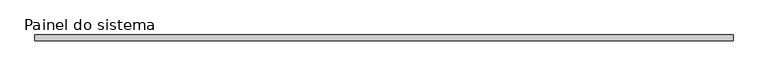
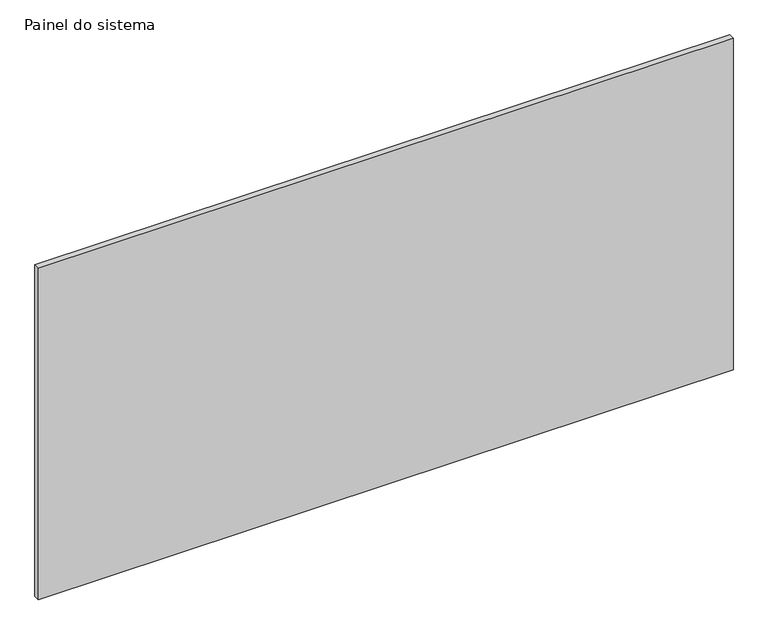
"""IFC4 building model written with IfcOpenShell, lengths in millimetres: plate geometry, Painel do sistema : Envidraçado."""

from ifc_helpers import new_model, si_unit, origin, origin_with_axes, place, context, project, spatial, polyline, outline, extrude, source, transform, mapped, element, save


def painel_do_sistema_ee4f1c4d(model_context):
    return source(origin(), model_context, "Body", "SweptSolid", [
        extrude(outline(polyline([(1487.5000075, 24.5), (-1487.5000075, 24.5), (-1487.5000075, 49.5), (1487.5000075, 49.5), (1487.5000075, 24.5)])), origin_with_axes(), (0.0, 0.0, 1.0), 1500.0),
    ])


if __name__ == "__main__":
    model = new_model("IFC4")
    model_context = context("Model", 3, world=origin())
    ifc_project = project(units=[si_unit("LENGTHUNIT", "METRE", prefix="MILLI")], contexts=[model_context])
    site = spatial("IfcSite", under=ifc_project)
    building = spatial("IfcBuilding", under=site)
    placement = place(None, origin())
    painel_do_sistema_shape = painel_do_sistema_ee4f1c4d(model_context)
    element("IfcPlate", 1, ObjectType="Painel do sistema : Envidraçado", at=placement, inside=building, context=model_context, shape_type="MappedRepresentation", body=[
        mapped(painel_do_sistema_shape, transform((0.0, 0.0, 0.0), x_axis=(1.0, 0.0, 0.0), y_axis=(0.0, 1.0, 0.0), z_axis=(0.0, 0.0, 1.0))),
    ])
    save(model, "model.ifc")

# Revit data of these elements
# Type "Painel do sistema : Envidraçado"
#   Construction Type Id = "GSP4R"
#   Analytic Construction = "Vidraça única Pilkington 1/8 pol"
#   Visual Light Transmittance = 0.9
#   Solar Heat Gain Coefficient = 0.86
#   Heat Transfer Coefficient (U) = 6.7069 W/(m²·K)
# Element 1 (IfcPlate, "Painel do sistema : Envidraçado")
#   Materials on its faces: "Vidro"
# Materials
#   "Vidro": class "Vidro", colour RGB 0 128 192, transparency 0.9, Description = "Vidro de sílica", Cost = 0
